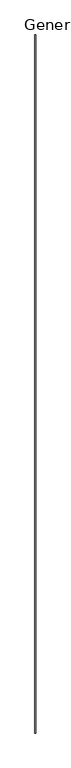
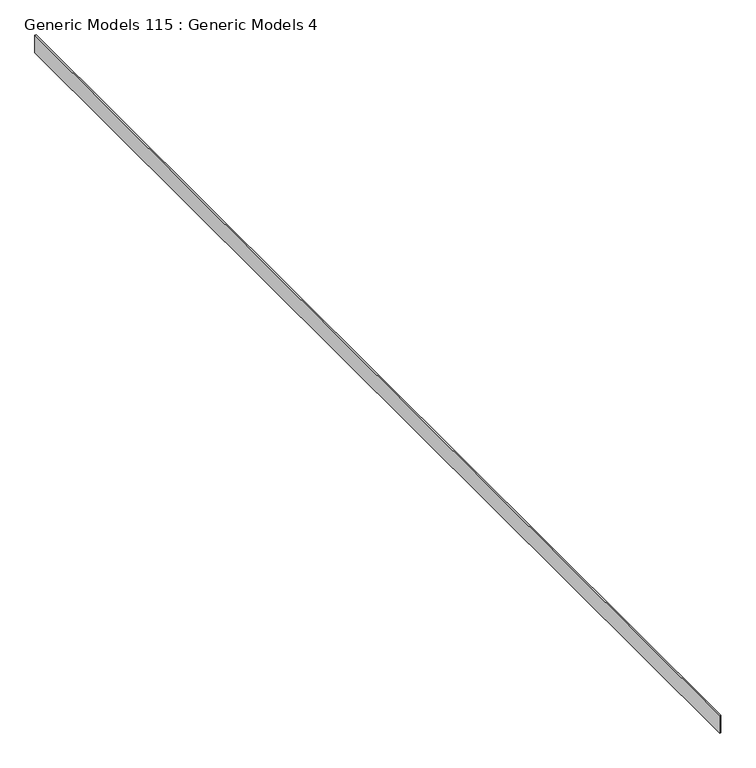
"""IFC4 building model written with IfcOpenShell, lengths in millimetres: proxy geometry, Generic Models 115 : Generic Models 4."""

from ifc_helpers import new_model, si_unit, frame, origin, place, context, project, spatial, polyline, outline, extrude, source, transform, mapped, element, save


def generic_models_115_generic_models_4_6853b713(model_context):
    return source(origin(), model_context, "Body", "SweptSolid", [
        extrude(outline(polyline([(7253.8514146, -6864.9230338), (7234.8014146, -6864.9230338), (7234.8014146, 11778.6769662), (7253.8514146, 11778.6769662), (7253.8514146, -6864.9230338)])), frame((0.0, 0.0, 126809.341198), z_axis=(0.0, 0.0, 1.0), x_axis=(1.0, 0.0, 0.0)), (0.0, 0.0, 1.0), 290.7625207),
    ])


if __name__ == "__main__":
    model = new_model("IFC4")
    model_context = context("Model", 3, world=origin())
    ifc_project = project(units=[si_unit("LENGTHUNIT", "METRE", prefix="MILLI")], contexts=[model_context])
    site = spatial("IfcSite", under=ifc_project)
    building = spatial("IfcBuilding", under=site)
    placement = place(None, origin())
    generic_models_115_generic_models_4_shape = generic_models_115_generic_models_4_6853b713(model_context)
    element("IfcBuildingElementProxy", 1, Name="Generic Models 115 : Generic Models 4", ObjectType="Generic Models 115 : Generic Models 4", at=placement, inside=building, context=model_context, shape_type="MappedRepresentation", body=[
        mapped(generic_models_115_generic_models_4_shape, transform((0.0, 0.0, 0.0), x_axis=(1.0, 0.0, 0.0), y_axis=(0.0, 1.0, 0.0), z_axis=(0.0, 0.0, 1.0))),
    ])
    save(model, "model.ifc")

# Revit data of these elements
# Element 1 (IfcBuildingElementProxy, "Generic Models 115 : Generic Models 4")
#   Materials on its faces: "_CDX PLYWOOD - SEE STRUCT DWGs"
# Materials
#   "_CDX PLYWOOD - SEE STRUCT DWGs": class "Generic", colour RGB 98 75 74, transparency 0, Cost = 0
